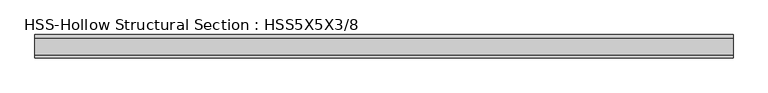
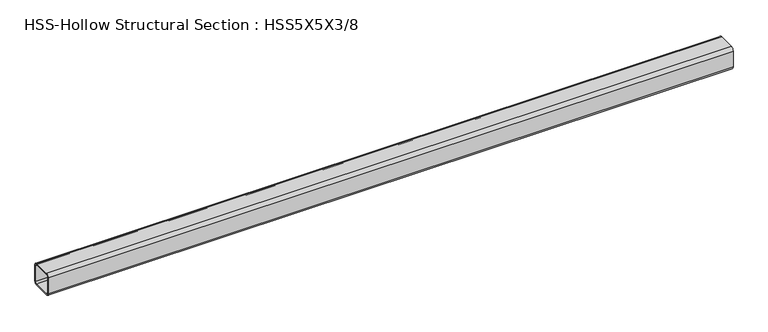
"""IFC4 building model written with IfcOpenShell, lengths in millimetres: member geometry, HSS-Hollow Structural Section : HSS5X5X3/8."""

import ifcopenshell
import ifcopenshell.guid

model = None  # the IFC model being written
_history = None  # IfcOwnerHistory: only IFC2X3 demands one
_inside = {}  # id of a spatial element -> (the spatial element, [elements in it])
_under = {}  # id of a project, library or spatial element -> (it, [spatial elements below it])
_declared = {}  # id of a project -> (the project, [libraries it declares])
_typed = {}  # id of a type object -> (the type object, [elements of that type])
_made_of = {}  # id of a material, layer set ... -> (it, [elements and type objects made of it])


def new_model(schema):
    """Start an empty IFC model of exactly this schema.

    Asked for "IFC4X3", IfcOpenShell would pick the latest addendum, in which some entities
    have other attributes; the version numbers below select the first issue.
    IFC2X3 requires an IfcOwnerHistory on every rooted entity: one is made here for all.
    """
    global model, _history
    if schema == "IFC4X3":
        model = ifcopenshell.file(schema_version=(4, 3, 0, 0))
    else:
        model = ifcopenshell.file(schema=schema)
    _inside.clear()
    _under.clear()
    _declared.clear()
    _typed.clear()
    _made_of.clear()
    _history = None
    if model.schema == "IFC2X3":
        org = make("IfcOrganization", Name="unknown")
        user = make(
            "IfcPersonAndOrganization",
            ThePerson=make("IfcPerson", FamilyName="unknown"),
            TheOrganization=org,
        )
        app = make(
            "IfcApplication",
            ApplicationDeveloper=org,
            Version="unknown",
            ApplicationFullName="unknown",
            ApplicationIdentifier="unknown",
        )
        _history = make(
            "IfcOwnerHistory",
            OwningUser=user,
            OwningApplication=app,
            ChangeAction="ADDED",
            CreationDate=0,
        )
    return model


def make(cls, **values):
    """One entity of the class cls with the attributes given. An attribute that is None is left unset."""
    return model.create_entity(
        cls, **{name: value for name, value in values.items() if value is not None}
    )


def rooted(cls, **values):
    """An entity with a GlobalId (a new one), such as an element, a storey or a relation."""
    return make(cls, GlobalId=ifcopenshell.guid.new(), OwnerHistory=_history, **values)


def si_unit(unit_type, name, prefix=None):
    """IfcSIUnit, for example si_unit("LENGTHUNIT", "METRE", prefix="MILLI")."""
    return make("IfcSIUnit", UnitType=unit_type, Prefix=prefix, Name=name)


def assignment(units):
    """IfcUnitAssignment: the units of a project."""
    return None if units is None else make("IfcUnitAssignment", Units=units)


def point(xyz):
    """IfcCartesianPoint."""
    return None if xyz is None else make("IfcCartesianPoint", Coordinates=xyz)


def direction(xyz):
    """IfcDirection."""
    return None if xyz is None else make("IfcDirection", DirectionRatios=xyz)


def frame(location, z_axis=None, x_axis=None):
    """IfcAxis2Placement3D, a coordinate frame: its origin and axes. An axis left out is left unset."""
    return make(
        "IfcAxis2Placement3D",
        Location=point(location),
        Axis=direction(z_axis),
        RefDirection=direction(x_axis),
    )


def frame_2d(location, x_axis=None):
    """IfcAxis2Placement2D, a coordinate frame in the plane: its origin and x axis."""
    return make(
        "IfcAxis2Placement2D", Location=point(location), RefDirection=direction(x_axis)
    )


def origin():
    """The frame at (0, 0, 0) with its axes left unset."""
    return frame((0.0, 0.0, 0.0))


def place(relative_to, where):
    """IfcLocalPlacement: puts the frame where relative to a parent placement (None: the world)."""
    return make(
        "IfcLocalPlacement", PlacementRelTo=relative_to, RelativePlacement=where
    )


def context(
    kind, dimensions, precision=None, world=None, true_north=None, identifier=None
):
    """IfcGeometricRepresentationContext, for example the 3D "Model" context."""
    return make(
        "IfcGeometricRepresentationContext",
        ContextIdentifier=identifier,
        ContextType=kind,
        CoordinateSpaceDimension=dimensions,
        Precision=precision,
        WorldCoordinateSystem=world,
        TrueNorth=true_north,
    )


def project(units=None, contexts=None):
    """IfcProject with its units and contexts."""
    return rooted(
        "IfcProject",
        Name="project",
        RepresentationContexts=contexts,
        UnitsInContext=assignment(units),
    )


def spatial(cls, under=None, at=None, **own):
    """A site, building, storey or space (cls), placed at a placement, below another one or the project."""
    s = rooted(cls, ObjectPlacement=at, **own)
    if under is not None:
        _under.setdefault(under.id(), (under, []))[1].append(s)
    return s


def polyline(points):
    """IfcPolyline through the points."""
    return make("IfcPolyline", Points=[point(p) for p in points])


def circle_curve(where, radius):
    """IfcCircle in the frame where."""
    return make("IfcCircle", Position=where, Radius=radius)


def trimmed(basis, trim1, trim2, sense, master):
    """IfcTrimmedCurve: the piece of a basis curve between two trims."""
    return make(
        "IfcTrimmedCurve",
        BasisCurve=basis,
        Trim1=trim1,
        Trim2=trim2,
        SenseAgreement=sense,
        MasterRepresentation=master,
    )


def segment(curve, same_sense, transition):
    """IfcCompositeCurveSegment."""
    return make(
        "IfcCompositeCurveSegment",
        Transition=transition,
        SameSense=same_sense,
        ParentCurve=curve,
    )


def composite_curve(segments, self_intersect=None):
    """IfcCompositeCurve: segments joined end to end."""
    return make("IfcCompositeCurve", Segments=segments, SelfIntersect=self_intersect)


def outline(outer, holes=None, kind="AREA"):
    """IfcArbitraryClosedProfileDef: a profile drawn as a closed curve; with holes, ...WithVoids."""
    if holes is None:
        return make("IfcArbitraryClosedProfileDef", ProfileType=kind, OuterCurve=outer)
    return make(
        "IfcArbitraryProfileDefWithVoids",
        ProfileType=kind,
        OuterCurve=outer,
        InnerCurves=holes,
    )


def extrude(swept, where, along, depth):
    """IfcExtrudedAreaSolid: the profile swept, set in the frame where, extruded along a direction by depth."""
    return make(
        "IfcExtrudedAreaSolid",
        SweptArea=swept,
        Position=where,
        ExtrudedDirection=direction(along),
        Depth=depth,
    )


def shape(context_of_items, identifier, shape_type, items):
    """IfcShapeRepresentation: the items that make up one representation, for example the "Body"."""
    return make(
        "IfcShapeRepresentation",
        ContextOfItems=context_of_items,
        RepresentationIdentifier=identifier,
        RepresentationType=shape_type,
        Items=items,
    )


def source(mapping_origin, context_of_items, identifier, shape_type, items):
    """IfcRepresentationMap: a shape defined once, which mapped items show again and again."""
    return make(
        "IfcRepresentationMap",
        MappingOrigin=mapping_origin,
        MappedRepresentation=shape(context_of_items, identifier, shape_type, items),
    )


def transform(
    local_origin,
    x_axis=None,
    y_axis=None,
    z_axis=None,
    scale=None,
    scale2=None,
    scale3=None,
    uniform=True,
):
    """IfcCartesianTransformationOperator3D, or its non-uniform kind. x_axis, y_axis, z_axis: its Axis1, 2, 3."""
    if uniform:
        return make(
            "IfcCartesianTransformationOperator3D",
            Axis1=direction(x_axis),
            Axis2=direction(y_axis),
            LocalOrigin=point(local_origin),
            Scale=scale,
            Axis3=direction(z_axis),
        )
    return make(
        "IfcCartesianTransformationOperator3DnonUniform",
        Axis1=direction(x_axis),
        Axis2=direction(y_axis),
        LocalOrigin=point(local_origin),
        Scale=scale,
        Axis3=direction(z_axis),
        Scale2=scale2,
        Scale3=scale3,
    )


def mapped(mapping_source, mapping_target):
    """IfcMappedItem: shows the shape of a source again, moved by a transform."""
    return make(
        "IfcMappedItem", MappingSource=mapping_source, MappingTarget=mapping_target
    )


def made_of(thing, what):
    """Note that an element or type object is made of a material, layer set ...; save() writes the relation."""
    if what is not None:
        _made_of.setdefault(what.id(), (what, []))[1].append(thing)
    return thing


def element(
    cls,
    number,
    at=None,
    inside=None,
    cuts=None,
    type_object=None,
    material=None,
    context=None,
    identifier="Body",
    shape_type=None,
    held_by="IfcProductDefinitionShape",
    body=None,
    shapes=None,
    **own,
):
    """One element of the class cls, such as IfcWall. Its Tag is "e" and its number.

    at: its placement. inside: the storey or other place that contains it. cuts: it is an
    opening in that element (IfcRelVoidsElement). A single representation is given by context,
    identifier, shape_type and body (its items); several are given by shapes. held_by: the class
    of the entity that holds the representations. save() writes the other relations.
    """
    e = rooted(cls, Tag="e%d" % number, ObjectPlacement=at, **own)
    if body is not None:
        shapes = [shape(context, identifier, shape_type, body)]
    if shapes is not None:
        e.Representation = make(held_by, Representations=shapes)
    if inside is not None:
        _inside.setdefault(inside.id(), (inside, []))[1].append(e)
    if cuts is not None:
        rooted(
            "IfcRelVoidsElement", RelatingBuildingElement=cuts, RelatedOpeningElement=e
        )
    if type_object is not None:
        _typed.setdefault(type_object.id(), (type_object, []))[1].append(e)
    return made_of(e, material)


def aggregate(whole, parts):
    """IfcRelAggregates: a whole, such as a stair, and the parts it consists of."""
    return rooted("IfcRelAggregates", RelatingObject=whole, RelatedObjects=parts)


def save(model, path):
    """Write the relations noted so far, then the file.

    IfcRelAggregates (storeys below a building ...), IfcRelContainedInSpatialStructure (elements
    in a storey), IfcRelDefinesByType, IfcRelAssociatesMaterial and IfcRelDeclares: one each for
    every whole, place, type object, material and project.
    """
    for whole, parts in _under.values():
        aggregate(whole, parts)
    for where, things in _inside.values():
        rooted(
            "IfcRelContainedInSpatialStructure",
            RelatedElements=things,
            RelatingStructure=where,
        )
    for kind, things in _typed.values():
        rooted("IfcRelDefinesByType", RelatedObjects=things, RelatingType=kind)
    for what, things in _made_of.values():
        rooted("IfcRelAssociatesMaterial", RelatedObjects=things, RelatingMaterial=what)
    for by, libraries in _declared.values():
        rooted("IfcRelDeclares", RelatingContext=by, RelatedDefinitions=libraries)
    model.write(path)


def hss_hollow_structural_section_hss5x5x3_8_86113892(model_context):
    return source(origin(), model_context, "Body", "SweptSolid", [
        extrude(outline(composite_curve([segment(polyline([(63.5, 45.7708), (63.5, -45.7708)]), True, "CONTINUOUS"), segment(trimmed(circle_curve(frame_2d((45.7708, -45.7708)), 17.7292), [point((63.5, -45.7708))], [point((45.7708, -63.5))], False, "CARTESIAN"), True, "CONTINUOUS"), segment(polyline([(45.7708, -63.5), (-45.7708, -63.5)]), True, "CONTINUOUS"), segment(trimmed(circle_curve(frame_2d((-45.7708, -45.7708)), 17.7292), [point((-45.7708, -63.5))], [point((-63.5, -45.7708))], False, "CARTESIAN"), True, "CONTINUOUS"), segment(polyline([(-63.5, -45.7708), (-63.5, 45.7708)]), True, "CONTINUOUS"), segment(trimmed(circle_curve(frame_2d((-45.7708, 45.7708)), 17.7292), [point((-63.5, 45.7708))], [point((-45.7708, 63.5))], False, "CARTESIAN"), True, "CONTINUOUS"), segment(polyline([(-45.7708, 63.5), (45.7708, 63.5)]), True, "CONTINUOUS"), segment(trimmed(circle_curve(frame_2d((45.7708, 45.7708)), 17.7292), [point((45.7708, 63.5))], [point((63.5, 45.7708))], False, "CARTESIAN"), True, "CONTINUOUS")], self_intersect=False), holes=[composite_curve([segment(trimmed(circle_curve(frame_2d((-45.7708, 45.7708)), 8.8646), [point((-45.7708, 54.6354))], [point((-54.6354, 45.7708))], True, "CARTESIAN"), True, "CONTINUOUS"), segment(polyline([(-54.6354, 45.7708), (-54.6354, -45.7708)]), True, "CONTINUOUS"), segment(trimmed(circle_curve(frame_2d((-45.7708, -45.7708)), 8.8646), [point((-54.6354, -45.7708))], [point((-45.7708, -54.6354))], True, "CARTESIAN"), True, "CONTINUOUS"), segment(polyline([(-45.7708, -54.6354), (45.7708, -54.6354)]), True, "CONTINUOUS"), segment(trimmed(circle_curve(frame_2d((45.7708, -45.7708)), 8.8646), [point((45.7708, -54.6354))], [point((54.6354, -45.7708))], True, "CARTESIAN"), True, "CONTINUOUS"), segment(polyline([(54.6354, -45.7708), (54.6354, 45.7708)]), True, "CONTINUOUS"), segment(trimmed(circle_curve(frame_2d((45.7708, 45.7708)), 8.8646), [point((54.6354, 45.7708))], [point((45.7708, 54.6354))], True, "CARTESIAN"), True, "CONTINUOUS"), segment(polyline([(45.7708, 54.6354), (-45.7708, 54.6354)]), True, "CONTINUOUS")], self_intersect=False)]), frame((-1783.4477506, 0.0, 0.0), z_axis=(1.0, 0.0, 0.0), x_axis=(0.0, 1.0, 0.0)), (0.0, 0.0, 1.0), 3778.090058),
    ])


if __name__ == "__main__":
    model = new_model("IFC4")
    model_context = context("Model", 3, world=origin())
    ifc_project = project(units=[si_unit("LENGTHUNIT", "METRE", prefix="MILLI")], contexts=[model_context])
    site = spatial("IfcSite", under=ifc_project)
    building = spatial("IfcBuilding", under=site)
    placement = place(None, origin())
    hss_hollow_structural_section_hss5x5x3_8_shape = hss_hollow_structural_section_hss5x5x3_8_86113892(model_context)
    element("IfcMember", 1, ObjectType="HSS-Hollow Structural Section : HSS5X5X3/8", at=placement, inside=building, context=model_context, shape_type="MappedRepresentation", body=[
        mapped(hss_hollow_structural_section_hss5x5x3_8_shape, transform((0.0, 0.0, 0.0), x_axis=(1.0, 0.0, 0.0), y_axis=(0.0, 1.0, 0.0), z_axis=(0.0, 0.0, 1.0))),
    ])
    save(model, "model.ifc")

# Revit data of these elements
# Type "HSS-Hollow Structural Section : HSS5X5X3/8"
#   Assembly Code = "B10"
#   Shape = "Square"
#   W = 22.3
#   Ht = 0' - 5"
#   Length [instance default] = 5' - 0"
#   b = 0' - 5"
#   kr = 0' - 0.698"
#   t = 0' - 0.349"
#   A = 0.0429167 SF
#   Structural Material [instance default] = Steel ASTM A500, Grade B, Rectangular and Square
# Element 1 (IfcMember, "HSS-Hollow Structural Section : HSS5X5X3/8")
#   Materials on its faces: "Steel ASTM A500, Grade B, Rectangular and Square"
# Materials
#   "Steel ASTM A500, Grade B, Rectangular and Square": class "Metal", colour RGB 199 199 199, transparency 0, Description = "Carbon steel", Cost = 0
